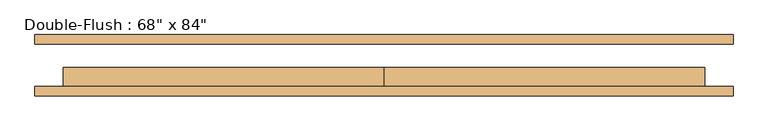
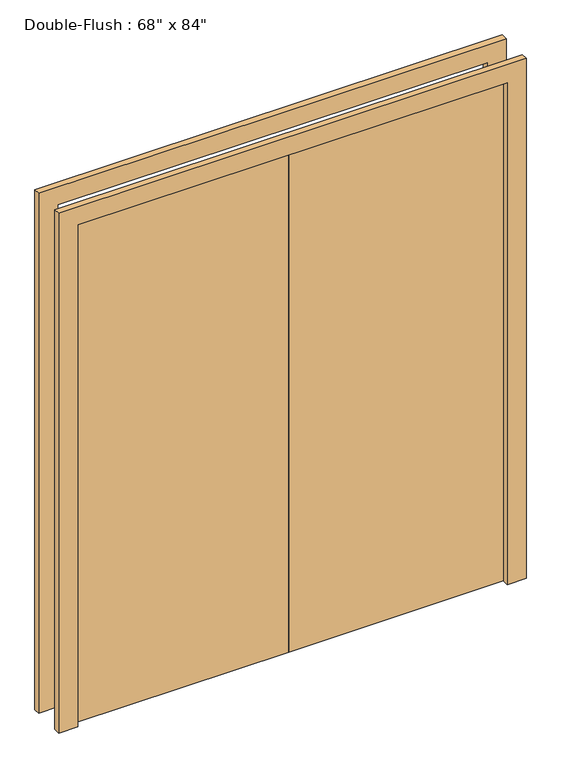
"""IFC4 building model written with IfcOpenShell, lengths in millimetres: door geometry."""

from ifc_helpers import new_model, si_unit, frame, origin, origin_with_axes, place, context, project, spatial, polyline, outline, extrude, source, transform, mapped, element, save


def door_63ee19b0(model_context):
    return source(origin(), model_context, "Body", "SweptSolid", [
        extrude(outline(polyline([(0.0, -57.15), (0.0, -6.35), (863.6, -6.35), (863.6, -57.15), (0.0, -57.15)])), origin_with_axes(), (0.0, 0.0, 1.0), 2133.6),
        extrude(outline(polyline([(-863.6, -57.15), (-863.6, -6.35), (0.0, -6.35), (0.0, -57.15), (-863.6, -57.15)])), origin_with_axes(), (0.0, 0.0, 1.0), 2133.6),
        extrude(outline(polyline([(2133.6, -863.6), (2133.6, 863.6), (0.0, 863.6), (0.0, 939.8), (2209.8, 939.8), (2209.8, -939.8), (0.0, -939.8), (0.0, -863.6), (2133.6, -863.6)])), frame((0.0, 57.15, 0.0), z_axis=(0.0, 1.0, 0.0), x_axis=(0.0, 0.0, 1.0)), (0.0, 0.0, 1.0), 25.4),
        extrude(outline(polyline([(2133.6, -863.6), (2133.6, 863.6), (0.0, 863.6), (0.0, 939.8), (2209.8, 939.8), (2209.8, -939.8), (0.0, -939.8), (0.0, -863.6), (2133.6, -863.6)])), frame((0.0, -82.55, 0.0), z_axis=(0.0, 1.0, 0.0), x_axis=(0.0, 0.0, 1.0)), (0.0, 0.0, 1.0), 25.4),
    ])


if __name__ == "__main__":
    model = new_model("IFC4")
    model_context = context("Model", 3, world=origin())
    ifc_project = project(units=[si_unit("LENGTHUNIT", "METRE", prefix="MILLI")], contexts=[model_context])
    site = spatial("IfcSite", under=ifc_project)
    building = spatial("IfcBuilding", under=site)
    placement = place(None, origin())
    door_shape = door_63ee19b0(model_context)
    element("IfcDoor", 1, ObjectType="Double-Flush : 68\" x 84\"", at=placement, inside=building, context=model_context, shape_type="MappedRepresentation", body=[
        mapped(door_shape, transform((0.0, 0.0, 0.0), x_axis=(1.0, 0.0, 0.0), y_axis=(0.0, 1.0, 0.0), z_axis=(0.0, 0.0, 1.0))),
    ])
    save(model, "model.ifc")

# Revit data of these elements
# Type "Double-Flush : 68\" x 84\""
#   Type Mark = "10"
#   Assembly Code = "C1020"
#   Thickness = 0' - 2"
#   Height = 7' - 0"
#   Trim Projection Ext = 0' - 1"
#   Trim Projection Int = 0' - 1"
#   Trim Width = 0' - 3"
#   Width = 5' - 8"
#   Function = 0
#   Door Material = Door - Panel
#   Frame Material = Door - Frame
#   Wall Closure = (empty or 0)
# Element 1 (IfcDoor, "Double-Flush : 68\" x 84\"")
#   Materials on its faces: "Door - Frame", "Door - Panel"
# Materials
#   "Door - Panel": class "Wood", colour RGB 210 159 95, transparency 0
#   "Door - Frame": class "Miscellaneous", colour RGB 118 70 51, transparency 0
